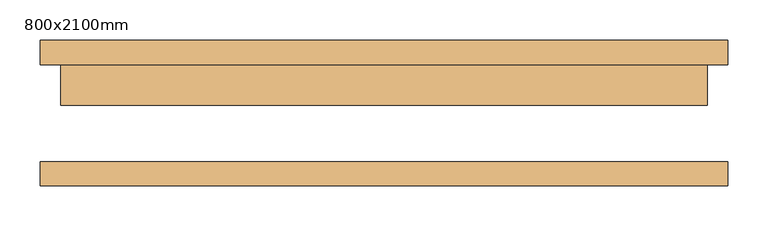
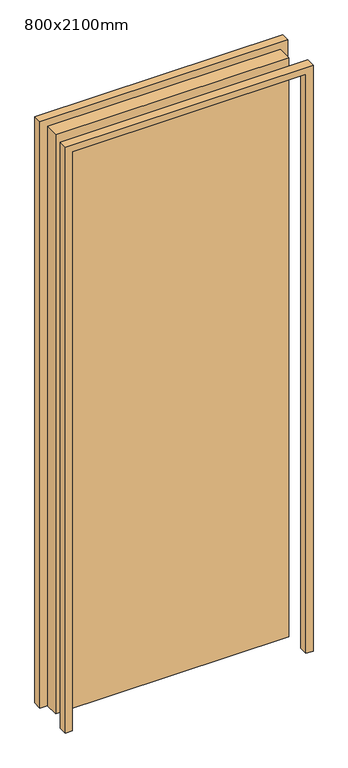
"""IFC4 building model written with IfcOpenShell, lengths in millimetres: door geometry, WWm-SingleSolid-Flush : 800x2100mm."""

import ifcopenshell
import ifcopenshell.guid

model = None  # the IFC model being written
_history = None  # IfcOwnerHistory: only IFC2X3 demands one
_inside = {}  # id of a spatial element -> (the spatial element, [elements in it])
_under = {}  # id of a project, library or spatial element -> (it, [spatial elements below it])
_declared = {}  # id of a project -> (the project, [libraries it declares])
_typed = {}  # id of a type object -> (the type object, [elements of that type])
_made_of = {}  # id of a material, layer set ... -> (it, [elements and type objects made of it])


def new_model(schema):
    """Start an empty IFC model of exactly this schema.

    Asked for "IFC4X3", IfcOpenShell would pick the latest addendum, in which some entities
    have other attributes; the version numbers below select the first issue.
    IFC2X3 requires an IfcOwnerHistory on every rooted entity: one is made here for all.
    """
    global model, _history
    if schema == "IFC4X3":
        model = ifcopenshell.file(schema_version=(4, 3, 0, 0))
    else:
        model = ifcopenshell.file(schema=schema)
    _inside.clear()
    _under.clear()
    _declared.clear()
    _typed.clear()
    _made_of.clear()
    _history = None
    if model.schema == "IFC2X3":
        org = make("IfcOrganization", Name="unknown")
        user = make(
            "IfcPersonAndOrganization",
            ThePerson=make("IfcPerson", FamilyName="unknown"),
            TheOrganization=org,
        )
        app = make(
            "IfcApplication",
            ApplicationDeveloper=org,
            Version="unknown",
            ApplicationFullName="unknown",
            ApplicationIdentifier="unknown",
        )
        _history = make(
            "IfcOwnerHistory",
            OwningUser=user,
            OwningApplication=app,
            ChangeAction="ADDED",
            CreationDate=0,
        )
    return model


def make(cls, **values):
    """One entity of the class cls with the attributes given. An attribute that is None is left unset."""
    return model.create_entity(
        cls, **{name: value for name, value in values.items() if value is not None}
    )


def rooted(cls, **values):
    """An entity with a GlobalId (a new one), such as an element, a storey or a relation."""
    return make(cls, GlobalId=ifcopenshell.guid.new(), OwnerHistory=_history, **values)


def si_unit(unit_type, name, prefix=None):
    """IfcSIUnit, for example si_unit("LENGTHUNIT", "METRE", prefix="MILLI")."""
    return make("IfcSIUnit", UnitType=unit_type, Prefix=prefix, Name=name)


def assignment(units):
    """IfcUnitAssignment: the units of a project."""
    return None if units is None else make("IfcUnitAssignment", Units=units)


def point(xyz):
    """IfcCartesianPoint."""
    return None if xyz is None else make("IfcCartesianPoint", Coordinates=xyz)


def direction(xyz):
    """IfcDirection."""
    return None if xyz is None else make("IfcDirection", DirectionRatios=xyz)


def frame(location, z_axis=None, x_axis=None):
    """IfcAxis2Placement3D, a coordinate frame: its origin and axes. An axis left out is left unset."""
    return make(
        "IfcAxis2Placement3D",
        Location=point(location),
        Axis=direction(z_axis),
        RefDirection=direction(x_axis),
    )


def origin():
    """The frame at (0, 0, 0) with its axes left unset."""
    return frame((0.0, 0.0, 0.0))


def origin_with_axes():
    """The frame at (0, 0, 0) with the z axis (0, 0, 1) and the x axis (1, 0, 0) written out."""
    return frame((0.0, 0.0, 0.0), z_axis=(0.0, 0.0, 1.0), x_axis=(1.0, 0.0, 0.0))


def place(relative_to, where):
    """IfcLocalPlacement: puts the frame where relative to a parent placement (None: the world)."""
    return make(
        "IfcLocalPlacement", PlacementRelTo=relative_to, RelativePlacement=where
    )


def context(
    kind, dimensions, precision=None, world=None, true_north=None, identifier=None
):
    """IfcGeometricRepresentationContext, for example the 3D "Model" context."""
    return make(
        "IfcGeometricRepresentationContext",
        ContextIdentifier=identifier,
        ContextType=kind,
        CoordinateSpaceDimension=dimensions,
        Precision=precision,
        WorldCoordinateSystem=world,
        TrueNorth=true_north,
    )


def project(units=None, contexts=None):
    """IfcProject with its units and contexts."""
    return rooted(
        "IfcProject",
        Name="project",
        RepresentationContexts=contexts,
        UnitsInContext=assignment(units),
    )


def spatial(cls, under=None, at=None, **own):
    """A site, building, storey or space (cls), placed at a placement, below another one or the project."""
    s = rooted(cls, ObjectPlacement=at, **own)
    if under is not None:
        _under.setdefault(under.id(), (under, []))[1].append(s)
    return s


def polyline(points):
    """IfcPolyline through the points."""
    return make("IfcPolyline", Points=[point(p) for p in points])


def outline(outer, holes=None, kind="AREA"):
    """IfcArbitraryClosedProfileDef: a profile drawn as a closed curve; with holes, ...WithVoids."""
    if holes is None:
        return make("IfcArbitraryClosedProfileDef", ProfileType=kind, OuterCurve=outer)
    return make(
        "IfcArbitraryProfileDefWithVoids",
        ProfileType=kind,
        OuterCurve=outer,
        InnerCurves=holes,
    )


def extrude(swept, where, along, depth):
    """IfcExtrudedAreaSolid: the profile swept, set in the frame where, extruded along a direction by depth."""
    return make(
        "IfcExtrudedAreaSolid",
        SweptArea=swept,
        Position=where,
        ExtrudedDirection=direction(along),
        Depth=depth,
    )


def shape(context_of_items, identifier, shape_type, items):
    """IfcShapeRepresentation: the items that make up one representation, for example the "Body"."""
    return make(
        "IfcShapeRepresentation",
        ContextOfItems=context_of_items,
        RepresentationIdentifier=identifier,
        RepresentationType=shape_type,
        Items=items,
    )


def source(mapping_origin, context_of_items, identifier, shape_type, items):
    """IfcRepresentationMap: a shape defined once, which mapped items show again and again."""
    return make(
        "IfcRepresentationMap",
        MappingOrigin=mapping_origin,
        MappedRepresentation=shape(context_of_items, identifier, shape_type, items),
    )


def transform(
    local_origin,
    x_axis=None,
    y_axis=None,
    z_axis=None,
    scale=None,
    scale2=None,
    scale3=None,
    uniform=True,
):
    """IfcCartesianTransformationOperator3D, or its non-uniform kind. x_axis, y_axis, z_axis: its Axis1, 2, 3."""
    if uniform:
        return make(
            "IfcCartesianTransformationOperator3D",
            Axis1=direction(x_axis),
            Axis2=direction(y_axis),
            LocalOrigin=point(local_origin),
            Scale=scale,
            Axis3=direction(z_axis),
        )
    return make(
        "IfcCartesianTransformationOperator3DnonUniform",
        Axis1=direction(x_axis),
        Axis2=direction(y_axis),
        LocalOrigin=point(local_origin),
        Scale=scale,
        Axis3=direction(z_axis),
        Scale2=scale2,
        Scale3=scale3,
    )


def mapped(mapping_source, mapping_target):
    """IfcMappedItem: shows the shape of a source again, moved by a transform."""
    return make(
        "IfcMappedItem", MappingSource=mapping_source, MappingTarget=mapping_target
    )


def made_of(thing, what):
    """Note that an element or type object is made of a material, layer set ...; save() writes the relation."""
    if what is not None:
        _made_of.setdefault(what.id(), (what, []))[1].append(thing)
    return thing


def element(
    cls,
    number,
    at=None,
    inside=None,
    cuts=None,
    type_object=None,
    material=None,
    context=None,
    identifier="Body",
    shape_type=None,
    held_by="IfcProductDefinitionShape",
    body=None,
    shapes=None,
    **own,
):
    """One element of the class cls, such as IfcWall. Its Tag is "e" and its number.

    at: its placement. inside: the storey or other place that contains it. cuts: it is an
    opening in that element (IfcRelVoidsElement). A single representation is given by context,
    identifier, shape_type and body (its items); several are given by shapes. held_by: the class
    of the entity that holds the representations. save() writes the other relations.
    """
    e = rooted(cls, Tag="e%d" % number, ObjectPlacement=at, **own)
    if body is not None:
        shapes = [shape(context, identifier, shape_type, body)]
    if shapes is not None:
        e.Representation = make(held_by, Representations=shapes)
    if inside is not None:
        _inside.setdefault(inside.id(), (inside, []))[1].append(e)
    if cuts is not None:
        rooted(
            "IfcRelVoidsElement", RelatingBuildingElement=cuts, RelatedOpeningElement=e
        )
    if type_object is not None:
        _typed.setdefault(type_object.id(), (type_object, []))[1].append(e)
    return made_of(e, material)


def aggregate(whole, parts):
    """IfcRelAggregates: a whole, such as a stair, and the parts it consists of."""
    return rooted("IfcRelAggregates", RelatingObject=whole, RelatedObjects=parts)


def save(model, path):
    """Write the relations noted so far, then the file.

    IfcRelAggregates (storeys below a building ...), IfcRelContainedInSpatialStructure (elements
    in a storey), IfcRelDefinesByType, IfcRelAssociatesMaterial and IfcRelDeclares: one each for
    every whole, place, type object, material and project.
    """
    for whole, parts in _under.values():
        aggregate(whole, parts)
    for where, things in _inside.values():
        rooted(
            "IfcRelContainedInSpatialStructure",
            RelatedElements=things,
            RelatingStructure=where,
        )
    for kind, things in _typed.values():
        rooted("IfcRelDefinesByType", RelatedObjects=things, RelatingType=kind)
    for what, things in _made_of.values():
        rooted("IfcRelAssociatesMaterial", RelatedObjects=things, RelatingMaterial=what)
    for by, libraries in _declared.values():
        rooted("IfcRelDeclares", RelatingContext=by, RelatedDefinitions=libraries)
    model.write(path)


def door_800x2100mm_99bb1da7(model_context):
    return source(origin(), model_context, "Body", "SweptSolid", [
        extrude(outline(polyline([(2125.0, -425.0), (0.0, -425.0), (0.0, -400.0), (2100.0, -400.0), (2100.0, 400.0), (0.0, 400.0), (0.0, 425.0), (2125.0, 425.0), (2125.0, -425.0)])), frame((0.0, 60.0, 0.0), z_axis=(0.0, 1.0, 0.0), x_axis=(0.0, 0.0, 1.0)), (0.0, 0.0, 1.0), 30.0),
        extrude(outline(polyline([(2125.0, 425.0), (2125.0, -425.0), (0.0, -425.0), (0.0, -400.0), (2100.0, -400.0), (2100.0, 400.0), (0.0, 400.0), (0.0, 425.0), (2125.0, 425.0)])), frame((0.0, -90.0, 0.0), z_axis=(0.0, 1.0, 0.0), x_axis=(0.0, 0.0, 1.0)), (0.0, 0.0, 1.0), 30.0),
        extrude(outline(polyline([(400.0, 10.0), (-400.0, 10.0), (-400.0, 60.0), (400.0, 60.0), (400.0, 10.0)])), origin_with_axes(), (0.0, 0.0, 1.0), 2100.0),
    ])


if __name__ == "__main__":
    model = new_model("IFC4")
    model_context = context("Model", 3, world=origin())
    ifc_project = project(units=[si_unit("LENGTHUNIT", "METRE", prefix="MILLI")], contexts=[model_context])
    site = spatial("IfcSite", under=ifc_project)
    building = spatial("IfcBuilding", under=site)
    placement = place(None, origin())
    door_800x2100mm_shape = door_800x2100mm_99bb1da7(model_context)
    element("IfcDoor", 1, ObjectType="WWm-SingleSolid-Flush : 800x2100mm", at=placement, inside=building, context=model_context, shape_type="MappedRepresentation", body=[
        mapped(door_800x2100mm_shape, transform((0.0, 0.0, 0.0), x_axis=(1.0, 0.0, 0.0), y_axis=(0.0, 1.0, 0.0), z_axis=(0.0, 0.0, 1.0))),
    ])
    save(model, "model.ifc")

# Revit data of these elements
# Type "WWm-SingleSolid-Flush : 800x2100mm"
#   Type Mark = "EX1-54"
#   Construction Type Id = "MDOOR"
#   Assembly Code = "C1020"
#   Analytic Construction = "Metal"
#   Thickness = 50 mm
#   Thermal Resistance (R) = 0.270117 (m²·K)/W
#   Heat Transfer Coefficient (U) = 3.7021 W/(m²·K)
#   Height = 2100 mm
#   Trim Projection Ext = 30 mm
#   Trim Projection Int = 30 mm
#   Trim Width = 25 mm
#   Width = 800 mm
#   Not 90 Degree [instance default] = no
#   90 Degree [instance default] = yes
#   Door Material = WW-EC-RGB-White
#   Frame Material = WW-EC-RGB-White
#   Visual Light Transmittance = 0
#   Solar Heat Gain Coefficient = 0
#   Function = (empty or 0)
#   Wall Closure = (empty or 0)
# Element 1 (IfcDoor, "WWm-SingleSolid-Flush : 800x2100mm")
#   Materials on its faces: "WW-EC-RGB-White"
# Materials
#   "WW-EC-RGB-White": class "Generic", colour RGB 255 255 255, transparency 0, Comments = "If region requests off-white, swith asset color to RGB 231-228-220", Description = "Generic Color", Cost = 0
